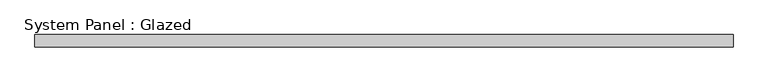
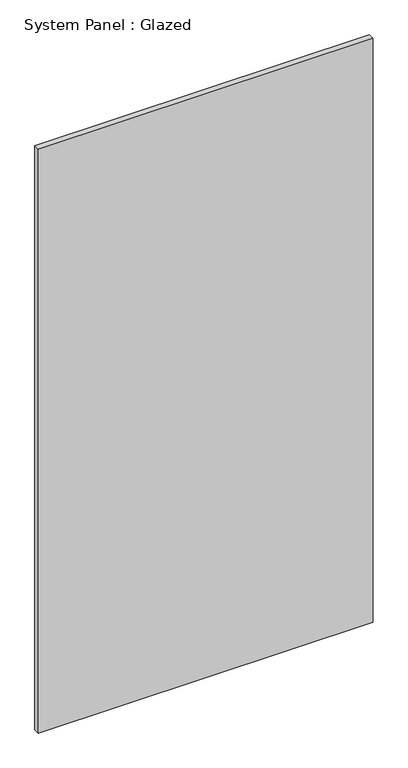
"""IFC4 building model written with IfcOpenShell, lengths in millimetres: plate geometry, System Panel : Glazed."""

import ifcopenshell
import ifcopenshell.guid

model = None  # the IFC model being written
_history = None  # IfcOwnerHistory: only IFC2X3 demands one
_inside = {}  # id of a spatial element -> (the spatial element, [elements in it])
_under = {}  # id of a project, library or spatial element -> (it, [spatial elements below it])
_declared = {}  # id of a project -> (the project, [libraries it declares])
_typed = {}  # id of a type object -> (the type object, [elements of that type])
_made_of = {}  # id of a material, layer set ... -> (it, [elements and type objects made of it])


def new_model(schema):
    """Start an empty IFC model of exactly this schema.

    Asked for "IFC4X3", IfcOpenShell would pick the latest addendum, in which some entities
    have other attributes; the version numbers below select the first issue.
    IFC2X3 requires an IfcOwnerHistory on every rooted entity: one is made here for all.
    """
    global model, _history
    if schema == "IFC4X3":
        model = ifcopenshell.file(schema_version=(4, 3, 0, 0))
    else:
        model = ifcopenshell.file(schema=schema)
    _inside.clear()
    _under.clear()
    _declared.clear()
    _typed.clear()
    _made_of.clear()
    _history = None
    if model.schema == "IFC2X3":
        org = make("IfcOrganization", Name="unknown")
        user = make(
            "IfcPersonAndOrganization",
            ThePerson=make("IfcPerson", FamilyName="unknown"),
            TheOrganization=org,
        )
        app = make(
            "IfcApplication",
            ApplicationDeveloper=org,
            Version="unknown",
            ApplicationFullName="unknown",
            ApplicationIdentifier="unknown",
        )
        _history = make(
            "IfcOwnerHistory",
            OwningUser=user,
            OwningApplication=app,
            ChangeAction="ADDED",
            CreationDate=0,
        )
    return model


def make(cls, **values):
    """One entity of the class cls with the attributes given. An attribute that is None is left unset."""
    return model.create_entity(
        cls, **{name: value for name, value in values.items() if value is not None}
    )


def rooted(cls, **values):
    """An entity with a GlobalId (a new one), such as an element, a storey or a relation."""
    return make(cls, GlobalId=ifcopenshell.guid.new(), OwnerHistory=_history, **values)


def si_unit(unit_type, name, prefix=None):
    """IfcSIUnit, for example si_unit("LENGTHUNIT", "METRE", prefix="MILLI")."""
    return make("IfcSIUnit", UnitType=unit_type, Prefix=prefix, Name=name)


def assignment(units):
    """IfcUnitAssignment: the units of a project."""
    return None if units is None else make("IfcUnitAssignment", Units=units)


def point(xyz):
    """IfcCartesianPoint."""
    return None if xyz is None else make("IfcCartesianPoint", Coordinates=xyz)


def direction(xyz):
    """IfcDirection."""
    return None if xyz is None else make("IfcDirection", DirectionRatios=xyz)


def frame(location, z_axis=None, x_axis=None):
    """IfcAxis2Placement3D, a coordinate frame: its origin and axes. An axis left out is left unset."""
    return make(
        "IfcAxis2Placement3D",
        Location=point(location),
        Axis=direction(z_axis),
        RefDirection=direction(x_axis),
    )


def origin():
    """The frame at (0, 0, 0) with its axes left unset."""
    return frame((0.0, 0.0, 0.0))


def origin_with_axes():
    """The frame at (0, 0, 0) with the z axis (0, 0, 1) and the x axis (1, 0, 0) written out."""
    return frame((0.0, 0.0, 0.0), z_axis=(0.0, 0.0, 1.0), x_axis=(1.0, 0.0, 0.0))


def place(relative_to, where):
    """IfcLocalPlacement: puts the frame where relative to a parent placement (None: the world)."""
    return make(
        "IfcLocalPlacement", PlacementRelTo=relative_to, RelativePlacement=where
    )


def context(
    kind, dimensions, precision=None, world=None, true_north=None, identifier=None
):
    """IfcGeometricRepresentationContext, for example the 3D "Model" context."""
    return make(
        "IfcGeometricRepresentationContext",
        ContextIdentifier=identifier,
        ContextType=kind,
        CoordinateSpaceDimension=dimensions,
        Precision=precision,
        WorldCoordinateSystem=world,
        TrueNorth=true_north,
    )


def project(units=None, contexts=None):
    """IfcProject with its units and contexts."""
    return rooted(
        "IfcProject",
        Name="project",
        RepresentationContexts=contexts,
        UnitsInContext=assignment(units),
    )


def spatial(cls, under=None, at=None, **own):
    """A site, building, storey or space (cls), placed at a placement, below another one or the project."""
    s = rooted(cls, ObjectPlacement=at, **own)
    if under is not None:
        _under.setdefault(under.id(), (under, []))[1].append(s)
    return s


def polyline(points):
    """IfcPolyline through the points."""
    return make("IfcPolyline", Points=[point(p) for p in points])


def outline(outer, holes=None, kind="AREA"):
    """IfcArbitraryClosedProfileDef: a profile drawn as a closed curve; with holes, ...WithVoids."""
    if holes is None:
        return make("IfcArbitraryClosedProfileDef", ProfileType=kind, OuterCurve=outer)
    return make(
        "IfcArbitraryProfileDefWithVoids",
        ProfileType=kind,
        OuterCurve=outer,
        InnerCurves=holes,
    )


def extrude(swept, where, along, depth):
    """IfcExtrudedAreaSolid: the profile swept, set in the frame where, extruded along a direction by depth."""
    return make(
        "IfcExtrudedAreaSolid",
        SweptArea=swept,
        Position=where,
        ExtrudedDirection=direction(along),
        Depth=depth,
    )


def shape(context_of_items, identifier, shape_type, items):
    """IfcShapeRepresentation: the items that make up one representation, for example the "Body"."""
    return make(
        "IfcShapeRepresentation",
        ContextOfItems=context_of_items,
        RepresentationIdentifier=identifier,
        RepresentationType=shape_type,
        Items=items,
    )


def source(mapping_origin, context_of_items, identifier, shape_type, items):
    """IfcRepresentationMap: a shape defined once, which mapped items show again and again."""
    return make(
        "IfcRepresentationMap",
        MappingOrigin=mapping_origin,
        MappedRepresentation=shape(context_of_items, identifier, shape_type, items),
    )


def transform(
    local_origin,
    x_axis=None,
    y_axis=None,
    z_axis=None,
    scale=None,
    scale2=None,
    scale3=None,
    uniform=True,
):
    """IfcCartesianTransformationOperator3D, or its non-uniform kind. x_axis, y_axis, z_axis: its Axis1, 2, 3."""
    if uniform:
        return make(
            "IfcCartesianTransformationOperator3D",
            Axis1=direction(x_axis),
            Axis2=direction(y_axis),
            LocalOrigin=point(local_origin),
            Scale=scale,
            Axis3=direction(z_axis),
        )
    return make(
        "IfcCartesianTransformationOperator3DnonUniform",
        Axis1=direction(x_axis),
        Axis2=direction(y_axis),
        LocalOrigin=point(local_origin),
        Scale=scale,
        Axis3=direction(z_axis),
        Scale2=scale2,
        Scale3=scale3,
    )


def mapped(mapping_source, mapping_target):
    """IfcMappedItem: shows the shape of a source again, moved by a transform."""
    return make(
        "IfcMappedItem", MappingSource=mapping_source, MappingTarget=mapping_target
    )


def made_of(thing, what):
    """Note that an element or type object is made of a material, layer set ...; save() writes the relation."""
    if what is not None:
        _made_of.setdefault(what.id(), (what, []))[1].append(thing)
    return thing


def element(
    cls,
    number,
    at=None,
    inside=None,
    cuts=None,
    type_object=None,
    material=None,
    context=None,
    identifier="Body",
    shape_type=None,
    held_by="IfcProductDefinitionShape",
    body=None,
    shapes=None,
    **own,
):
    """One element of the class cls, such as IfcWall. Its Tag is "e" and its number.

    at: its placement. inside: the storey or other place that contains it. cuts: it is an
    opening in that element (IfcRelVoidsElement). A single representation is given by context,
    identifier, shape_type and body (its items); several are given by shapes. held_by: the class
    of the entity that holds the representations. save() writes the other relations.
    """
    e = rooted(cls, Tag="e%d" % number, ObjectPlacement=at, **own)
    if body is not None:
        shapes = [shape(context, identifier, shape_type, body)]
    if shapes is not None:
        e.Representation = make(held_by, Representations=shapes)
    if inside is not None:
        _inside.setdefault(inside.id(), (inside, []))[1].append(e)
    if cuts is not None:
        rooted(
            "IfcRelVoidsElement", RelatingBuildingElement=cuts, RelatedOpeningElement=e
        )
    if type_object is not None:
        _typed.setdefault(type_object.id(), (type_object, []))[1].append(e)
    return made_of(e, material)


def aggregate(whole, parts):
    """IfcRelAggregates: a whole, such as a stair, and the parts it consists of."""
    return rooted("IfcRelAggregates", RelatingObject=whole, RelatedObjects=parts)


def save(model, path):
    """Write the relations noted so far, then the file.

    IfcRelAggregates (storeys below a building ...), IfcRelContainedInSpatialStructure (elements
    in a storey), IfcRelDefinesByType, IfcRelAssociatesMaterial and IfcRelDeclares: one each for
    every whole, place, type object, material and project.
    """
    for whole, parts in _under.values():
        aggregate(whole, parts)
    for where, things in _inside.values():
        rooted(
            "IfcRelContainedInSpatialStructure",
            RelatedElements=things,
            RelatingStructure=where,
        )
    for kind, things in _typed.values():
        rooted("IfcRelDefinesByType", RelatedObjects=things, RelatingType=kind)
    for what, things in _made_of.values():
        rooted("IfcRelAssociatesMaterial", RelatedObjects=things, RelatingMaterial=what)
    for by, libraries in _declared.values():
        rooted("IfcRelDeclares", RelatingContext=by, RelatedDefinitions=libraries)
    model.write(path)


def system_panel_glazed_ee6efdaa(model_context):
    return source(origin(), model_context, "Body", "SweptSolid", [
        extrude(outline(polyline([(712.5, -49.5), (-712.5, -49.5), (-712.5, -24.5), (712.5, -24.5), (712.5, -49.5)])), origin_with_axes(), (0.0, 0.0, 1.0), 2625.0),
    ])


if __name__ == "__main__":
    model = new_model("IFC4")
    model_context = context("Model", 3, world=origin())
    ifc_project = project(units=[si_unit("LENGTHUNIT", "METRE", prefix="MILLI")], contexts=[model_context])
    site = spatial("IfcSite", under=ifc_project)
    building = spatial("IfcBuilding", under=site)
    placement = place(None, origin())
    system_panel_glazed_shape = system_panel_glazed_ee6efdaa(model_context)
    element("IfcPlate", 1, ObjectType="System Panel : Glazed", at=placement, inside=building, context=model_context, shape_type="MappedRepresentation", body=[
        mapped(system_panel_glazed_shape, transform((0.0, 0.0, 0.0), x_axis=(1.0, 0.0, 0.0), y_axis=(0.0, 1.0, 0.0), z_axis=(0.0, 0.0, 1.0))),
    ])
    save(model, "model.ifc")

# Revit data of these elements
# Type "System Panel : Glazed"
#   Keynote = "H11"
#   Construction Type Id = "GSP4R"
#   Analytic Construction = "1/8 in Pilkington single glazing"
#   Visual Light Transmittance = 0.9
#   Solar Heat Gain Coefficient = 0.86
#   Heat Transfer Coefficient (U) = 6.7069 W/(m²·K)
# Element 1 (IfcPlate, "System Panel : Glazed")
#   Materials on its faces: "Glass"
# Materials
#   "Glass": class "Glass", colour RGB 0 128 192, transparency 0.9, Description = "Soda Lime Glass", Cost = 0
